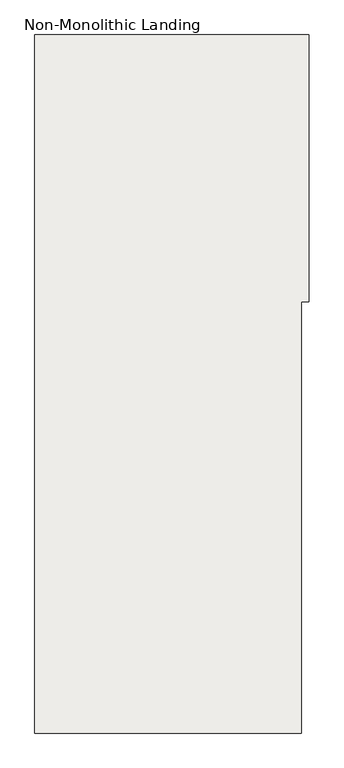
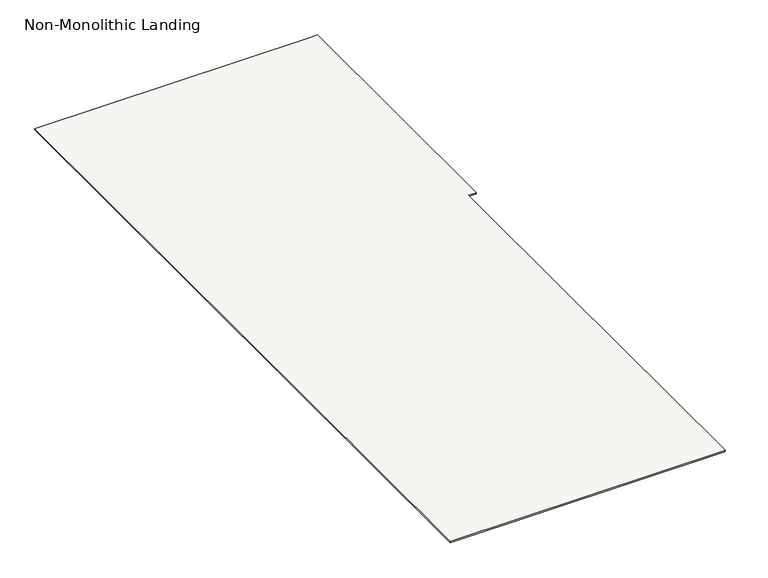
"""IFC4 building model written with IfcOpenShell, lengths in millimetres: slab geometry, Non-Monolithic Landing."""

from ifc_helpers import new_model, si_unit, origin, place, context, project, spatial, faceted_brep, source, transform, mapped, element, save


def non_monolithic_landing_09c0d781(model_context):
    return source(origin(), model_context, "Body", "Brep", [
        faceted_brep([(-16318.9400908, 12075.4345331, 22117.6470588), (-16318.0900908, 12075.4345331, 22111.6470588), (-16318.0900908, 13175.4345331, 22111.6470588), (-16318.9400908, 13175.4345331, 22117.6470588), (-16350.0, 11395.4345331, 22117.6470588), (-16350.0, 12075.4345331, 22117.6470588), (-16350.0, 13175.4345331, 22117.6470588), (-17450.0, 13175.4345331, 22117.6470588), (-17450.0, 10295.4345331, 22117.6470588), (-16350.0, 10295.4345331, 22117.6470588), (-16350.0, 12075.4345331, 22111.6470588), (-16350.0, 11395.4345331, 22111.6470588), (-16350.85, 11395.4345331, 22111.6470588), (-16350.85, 10295.4345331, 22111.6470588), (-17450.0, 10295.4345331, 22111.6470588), (-17450.0, 13175.4345331, 22111.6470588), (-16350.0, 13175.4345331, 22111.6470588)], [[[0, 1, 2, 3]], [[4, 5, 0, 3, 6, 7, 8, 9]], [[10, 11, 12, 13, 14, 15, 16, 2, 1]], [[5, 4, 11, 10]], [[0, 5, 10, 1]], [[6, 3, 2, 16]], [[7, 6, 16, 15]], [[8, 7, 15, 14]], [[9, 8, 14, 13]], [[4, 12, 11]], [[12, 4, 9, 13]]]),
    ])


if __name__ == "__main__":
    model = new_model("IFC4")
    model_context = context("Model", 3, world=origin())
    ifc_project = project(units=[si_unit("LENGTHUNIT", "METRE", prefix="MILLI")], contexts=[model_context])
    site = spatial("IfcSite", under=ifc_project)
    building = spatial("IfcBuilding", under=site)
    placement = place(None, origin())
    non_monolithic_landing_shape = non_monolithic_landing_09c0d781(model_context)
    element("IfcSlab", 1, ObjectType="Non-Monolithic Landing", at=placement, inside=building, context=model_context, shape_type="MappedRepresentation", body=[
        mapped(non_monolithic_landing_shape, transform((0.0, 0.0, 0.0), x_axis=(1.0, 0.0, 0.0), y_axis=(0.0, 1.0, 0.0), z_axis=(0.0, 0.0, 1.0))),
    ])
    save(model, "model.ifc")

# Revit data of these elements
# Element 1 (IfcSlab, "Non-Monolithic Landing")
#   Materials on its faces: "Steel, Paint Finish, Dark Gray"
# Materials
#   "Steel, Paint Finish, Dark Gray": class "Metal", colour RGB 89 89 89, transparency 0, Description = "Steel, paint finish, dark gray, glossy", Cost = 0
